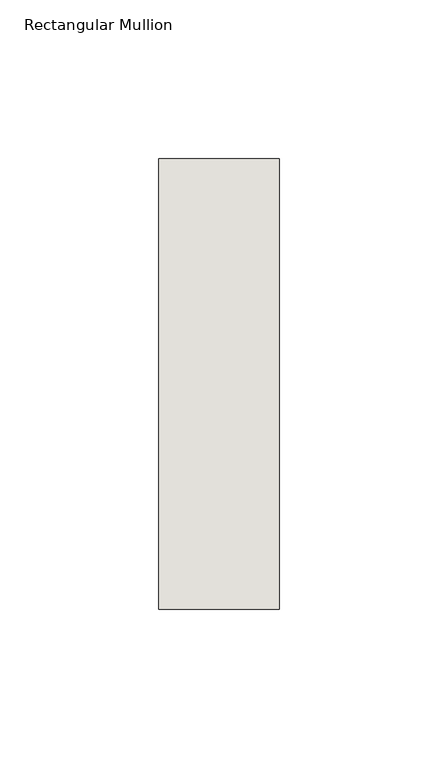
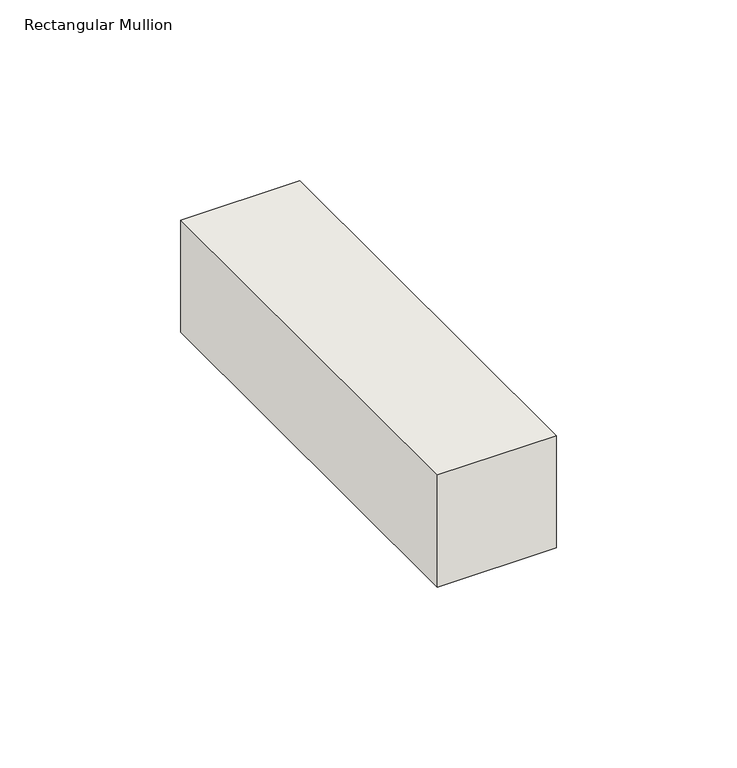
"""IFC4 building model written with IfcOpenShell, lengths in millimetres: wall geometry, Rectangular Mullion : NLRS_21_CWM_hsb-regel 38x142_gen_rsf."""

from ifc_helpers import new_model, si_unit, frame, origin, place, context, project, spatial, polyline, outline, extrude, source, transform, mapped, element, save


def rectangular_mullion_ad49c1d0(model_context):
    return source(origin(), model_context, "Body", "SweptSolid", [
        extrude(outline(polyline([(-38.0, -71.0), (-38.0, 71.0), (0.0, 71.0), (0.0, -71.0), (-38.0, -71.0)])), frame((0.0, 0.0, -38.0), z_axis=(0.0, 0.0, 1.0), x_axis=(1.0, 0.0, 0.0)), (0.0, 0.0, 1.0), 38.0),
    ])


if __name__ == "__main__":
    model = new_model("IFC4")
    model_context = context("Model", 3, world=origin())
    ifc_project = project(units=[si_unit("LENGTHUNIT", "METRE", prefix="MILLI")], contexts=[model_context])
    site = spatial("IfcSite", under=ifc_project)
    building = spatial("IfcBuilding", under=site)
    placement = place(None, origin())
    rectangular_mullion_shape = rectangular_mullion_ad49c1d0(model_context)
    element("IfcWall", 1, ObjectType="Rectangular Mullion : NLRS_21_CWM_hsb-regel 38x142_gen_rsf", at=placement, inside=building, context=model_context, shape_type="MappedRepresentation", body=[
        mapped(rectangular_mullion_shape, transform((0.0, 0.0, 0.0), x_axis=(1.0, 0.0, 0.0), y_axis=(0.0, 1.0, 0.0), z_axis=(0.0, 0.0, 1.0))),
    ])
    save(model, "model.ifc")

# Revit data of these elements
# Type "Rectangular Mullion : NLRS_21_CWM_hsb-regel 38x142_gen_rsf"
#   Type IfcGUID = "07M7mRoiH1CR8m_RSKIwpF"
#   Assembly Code = "21.10"
#   IfcExportAs = "IfcWall"
#   built-in parameter 1007322 = 0.465879 (stored number, unit not read)
#   built-in parameter 1007321 = 0.062336 (stored number, unit not read)
#   built-in parameter 1007320 = 0.062336 (stored number, unit not read)
# Element 1 (IfcWall, "Rectangular Mullion : NLRS_21_CWM_hsb-regel 38x142_gen_rsf")
#   Materials on its faces: "NLRS_i2_hout naaldhout vuren_gen_rsf"
# Materials
#   "NLRS_i2_hout naaldhout vuren_gen_rsf": class "I - Hout", colour RGB 234 199 147, transparency 0, Keynote = "i2", Manufacturer = "Revit Standards Foundation", URL = "www.revitstandards.org", Description = "hout vuren", Cost = 0
